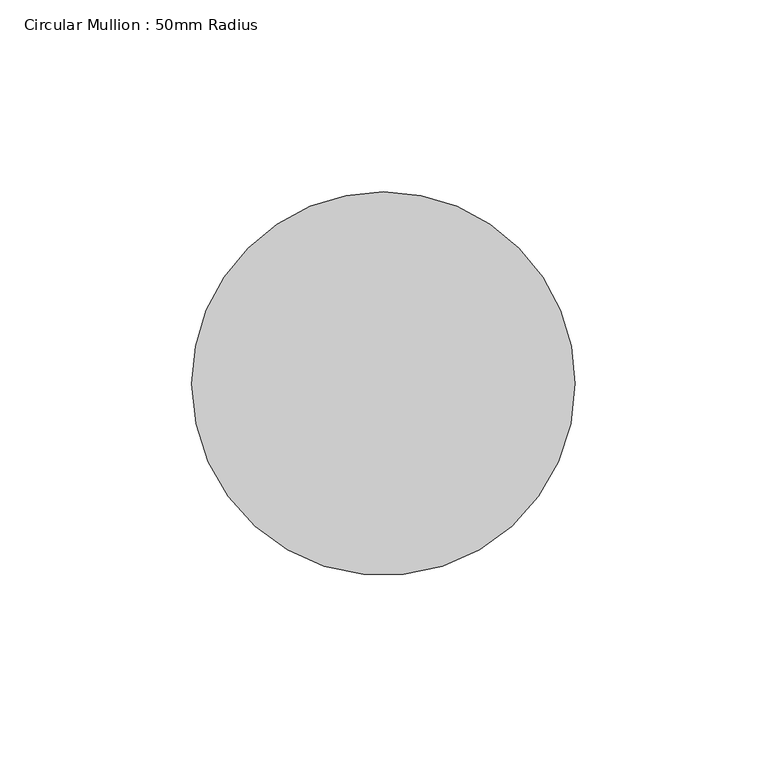
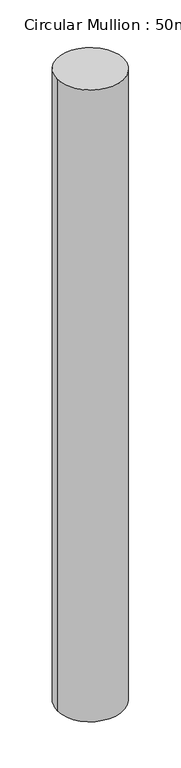
"""IFC4 building model written with IfcOpenShell, lengths in millimetres: member geometry, Circular Mullion : 50mm Radius."""

from ifc_helpers import new_model, si_unit, frame, origin, place, context, project, spatial, ellipse_curve, source, transform, mapped, element, save
from ifc_brep_helpers import plane_surface, cylinder_surface, advanced_brep


def circular_mullion_50mm_radius_10b3e52c(model_context):
    return source(origin(), model_context, "Body", "AdvancedBrep", [
        advanced_brep(
        [(-100.0, 0.0, 1.6710119), (0.0, 0.0, 0.0), (0.0, 0.0, -1006.1976773), (-100.0, 0.0, -1007.846805)],
        [
            (0, 1, ellipse_curve(frame((-50.0, 0.0, 0.8355059), z_axis=(-0.01670604325685514, -0.014444494501703127, -0.9997561026056757), x_axis=(-0.7562677305033517, -0.6538894283413674, 0.022084730080071197)), 50.0121978, 50.0)),
            (1, 2),
            (2, 3, ellipse_curve(frame((-50.0, 0.0, -1007.0222412), z_axis=(-0.016487359413510157, -0.014255414566722106, 0.9997624468518012), x_axis=(0.7562725296224475, 0.6538935777888973, 0.021795638666932775)), 50.0118805, 50.0)),
            (3, 0),
            (1, 0, ellipse_curve(frame((-50.0, 0.0, 0.8355059), z_axis=(-0.01670604325685514, -0.014444494501703127, -0.9997561026056757), x_axis=(-0.7562677305033517, -0.6538894283413674, 0.022084730080071197)), 50.0121978, 50.0)),
            (3, 2, ellipse_curve(frame((-50.0, 0.0, -1007.0222412), z_axis=(-0.016487359413510157, -0.014255414566722106, 0.9997624468518012), x_axis=(0.7562725296224475, 0.6538935777888973, 0.021795638666932775)), 50.0118805, 50.0)),
        ],
        [
            cylinder_surface(frame((-50.0, 0.0, 0.0), z_axis=(0.0, 0.0, 1.0), x_axis=(1.0, 0.0, 0.0)), 50.0),
            plane_surface(frame((-199.3541197, 230.5666389, 0.0), z_axis=(0.016706043256855145, 0.01444449450170313, 0.9997561026056759), x_axis=(0.7562677305033514, 0.6538894283413679, -0.02208473008007223))),
            plane_surface(frame((-199.3541197, 230.5666389, -1006.1976773), z_axis=(0.01648735941351016, 0.01425541456672211, -0.9997624468518014), x_axis=(0.7562725296224476, 0.6538935777888975, 0.021795638666930017))),
        ],
        [
            (0, [[1, 2, 3, 4]]),
            (0, [[5, -4, 6, -2]]),
            (1, [[-1, -5]]),
            (2, [[-6, -3]]),
        ],
    ),
    ])


if __name__ == "__main__":
    model = new_model("IFC4")
    model_context = context("Model", 3, world=origin())
    ifc_project = project(units=[si_unit("LENGTHUNIT", "METRE", prefix="MILLI")], contexts=[model_context])
    site = spatial("IfcSite", under=ifc_project)
    building = spatial("IfcBuilding", under=site)
    placement = place(None, origin())
    circular_mullion_50mm_radius_shape = circular_mullion_50mm_radius_10b3e52c(model_context)
    element("IfcMember", 1, ObjectType="Circular Mullion : 50mm Radius", at=placement, inside=building, context=model_context, shape_type="MappedRepresentation", body=[
        mapped(circular_mullion_50mm_radius_shape, transform((0.0, 0.0, 0.0), x_axis=(1.0, 0.0, 0.0), y_axis=(0.0, 1.0, 0.0), z_axis=(0.0, 0.0, 1.0))),
    ])
    save(model, "model.ifc")

# Revit data of these elements
# Type "Circular Mullion : 50mm Radius"
#   built-in parameter 1007350 = 0.164042 (stored number, unit not read)
# Element 1 (IfcMember, "Circular Mullion : 50mm Radius")
#   Materials on its faces: "Aluminium"
# Materials
#   "Aluminium": class "Metal", colour RGB 247 247 247, transparency 0, Description = "Aluminium 6061", Cost = 0
